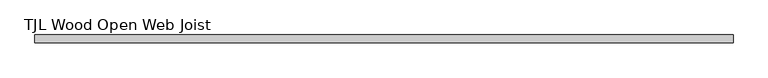
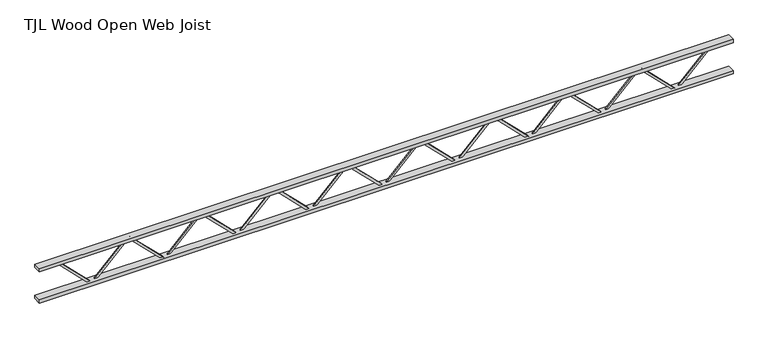
"""IFC4 building model written with IfcOpenShell, lengths in millimetres: beam geometry, TJL Wood Open Web Joist."""

from ifc_helpers import new_model, si_unit, frame, origin, place, context, project, spatial, polyline, outline, extrude, source, transform, mapped, element, save


def tjl_wood_open_web_joist_31244e6a(model_context):
    return source(origin(), model_context, "Body", "SweptSolid", [
        extrude(outline(polyline([(171.45, 2860.2340278), (196.85, 2860.2340278), (196.85, 2842.2957039), (-171.45, 2471.7908428), (-171.45, 2426.2291667), (-196.85, 2426.2291667), (-196.85, 2482.2674905), (171.45, 2852.7723517), (171.45, 2860.2340278)])), frame((0.0, 0.0, 0.0), z_axis=(0.0, 1.0, 0.0), x_axis=(0.0, 0.0, 1.0)), (0.0, 0.0, 1.0), 12.7),
        extrude(outline(polyline([(196.85, 2043.0243056), (171.45, 2043.0243056), (171.45, 2050.4859817), (-196.85, 2420.9908428), (-196.85, 2477.0291667), (-171.45, 2477.0291667), (-171.45, 2431.4674905), (196.85, 2060.9626294), (196.85, 2043.0243056)])), frame((0.0, -12.7, 0.0), z_axis=(0.0, 1.0, 0.0), x_axis=(0.0, 0.0, 1.0)), (0.0, 0.0, 1.0), 12.7),
        extrude(outline(polyline([(171.45, 2043.0243056), (196.85, 2043.0243056), (196.85, 2025.0859817), (-171.45, 1654.5811206), (-171.45, 1609.0194444), (-196.85, 1609.0194444), (-196.85, 1665.0577683), (171.45, 2035.5626294), (171.45, 2043.0243056)])), frame((0.0, 0.0, 0.0), z_axis=(0.0, 1.0, 0.0), x_axis=(0.0, 0.0, 1.0)), (0.0, 0.0, 1.0), 12.7),
        extrude(outline(polyline([(196.85, 1225.8145833), (171.45, 1225.8145833), (171.45, 1233.2762595), (-196.85, 1603.7811206), (-196.85, 1659.8194444), (-171.45, 1659.8194444), (-171.45, 1614.2577683), (196.85, 1243.7529072), (196.85, 1225.8145833)])), frame((0.0, -12.7, 0.0), z_axis=(0.0, 1.0, 0.0), x_axis=(0.0, 0.0, 1.0)), (0.0, 0.0, 1.0), 12.7),
        extrude(outline(polyline([(171.45, 1225.8145833), (196.85, 1225.8145833), (196.85, 1207.8762595), (-171.45, 837.3713983), (-171.45, 791.8097222), (-196.85, 791.8097222), (-196.85, 847.8480461), (171.45, 1218.3529072), (171.45, 1225.8145833)])), frame((0.0, 0.0, 0.0), z_axis=(0.0, 1.0, 0.0), x_axis=(0.0, 0.0, 1.0)), (0.0, 0.0, 1.0), 12.7),
        extrude(outline(polyline([(196.85, 408.6048611), (171.45, 408.6048611), (171.45, 416.0665372), (-196.85, 786.5713983), (-196.85, 842.6097222), (-171.45, 842.6097222), (-171.45, 797.0480461), (196.85, 426.543185), (196.85, 408.6048611)])), frame((0.0, -12.7, 0.0), z_axis=(0.0, 1.0, 0.0), x_axis=(0.0, 0.0, 1.0)), (0.0, 0.0, 1.0), 12.7),
        extrude(outline(polyline([(171.45, 408.6048611), (196.85, 408.6048611), (196.85, 390.6665372), (-171.45, 20.1616761), (-171.45, -25.4), (-196.85, -25.4), (-196.85, 30.6383239), (171.45, 401.143185), (171.45, 408.6048611)])), frame((0.0, 0.0, 0.0), z_axis=(0.0, 1.0, 0.0), x_axis=(0.0, 0.0, 1.0)), (0.0, 0.0, 1.0), 12.7),
        extrude(outline(polyline([(196.85, -408.6048611), (171.45, -408.6048611), (171.45, -401.143185), (-196.85, -30.6383239), (-196.85, 25.4), (-171.45, 25.4), (-171.45, -20.1616761), (196.85, -390.6665372), (196.85, -408.6048611)])), frame((0.0, -12.7, 0.0), z_axis=(0.0, 1.0, 0.0), x_axis=(0.0, 0.0, 1.0)), (0.0, 0.0, 1.0), 12.7),
        extrude(outline(polyline([(171.45, -408.6048611), (196.85, -408.6048611), (196.85, -426.543185), (-171.45, -797.0480461), (-171.45, -842.6097222), (-196.85, -842.6097222), (-196.85, -786.5713983), (171.45, -416.0665372), (171.45, -408.6048611)])), frame((0.0, 0.0, 0.0), z_axis=(0.0, 1.0, 0.0), x_axis=(0.0, 0.0, 1.0)), (0.0, 0.0, 1.0), 12.7),
        extrude(outline(polyline([(196.85, -1225.8145833), (171.45, -1225.8145833), (171.45, -1218.3529072), (-196.85, -847.8480461), (-196.85, -791.8097222), (-171.45, -791.8097222), (-171.45, -837.3713983), (196.85, -1207.8762595), (196.85, -1225.8145833)])), frame((0.0, -12.7, 0.0), z_axis=(0.0, 1.0, 0.0), x_axis=(0.0, 0.0, 1.0)), (0.0, 0.0, 1.0), 12.7),
        extrude(outline(polyline([(171.45, -1225.8145833), (196.85, -1225.8145833), (196.85, -1243.7529072), (-171.45, -1614.2577683), (-171.45, -1659.8194444), (-196.85, -1659.8194444), (-196.85, -1603.7811206), (171.45, -1233.2762595), (171.45, -1225.8145833)])), frame((0.0, 0.0, 0.0), z_axis=(0.0, 1.0, 0.0), x_axis=(0.0, 0.0, 1.0)), (0.0, 0.0, 1.0), 12.7),
        extrude(outline(polyline([(196.85, -2043.0243056), (171.45, -2043.0243056), (171.45, -2035.5626294), (-196.85, -1665.0577683), (-196.85, -1609.0194444), (-171.45, -1609.0194444), (-171.45, -1654.5811206), (196.85, -2025.0859817), (196.85, -2043.0243056)])), frame((0.0, -12.7, 0.0), z_axis=(0.0, 1.0, 0.0), x_axis=(0.0, 0.0, 1.0)), (0.0, 0.0, 1.0), 12.7),
        extrude(outline(polyline([(171.45, -2043.0243056), (196.85, -2043.0243056), (196.85, -2060.9626294), (-171.45, -2431.4674905), (-171.45, -2477.0291667), (-196.85, -2477.0291667), (-196.85, -2420.9908428), (171.45, -2050.4859817), (171.45, -2043.0243056)])), frame((0.0, 0.0, 0.0), z_axis=(0.0, 1.0, 0.0), x_axis=(0.0, 0.0, 1.0)), (0.0, 0.0, 1.0), 12.7),
        extrude(outline(polyline([(196.85, -2860.2340278), (171.45, -2860.2340278), (171.45, -2852.7723517), (-196.85, -2482.2674905), (-196.85, -2426.2291667), (-171.45, -2426.2291667), (-171.45, -2471.7908428), (196.85, -2842.2957039), (196.85, -2860.2340278)])), frame((0.0, -12.7, 0.0), z_axis=(0.0, 1.0, 0.0), x_axis=(0.0, 0.0, 1.0)), (0.0, 0.0, 1.0), 12.7),
        extrude(outline(polyline([(171.45, 3677.44375), (196.85, 3677.44375), (196.85, 3659.5054261), (-171.45, 3289.000565), (-171.45, 3243.4388889), (-196.85, 3243.4388889), (-196.85, 3299.4772128), (171.45, 3669.9820739), (171.45, 3677.44375)])), frame((0.0, 0.0, 0.0), z_axis=(0.0, 1.0, 0.0), x_axis=(0.0, 0.0, 1.0)), (0.0, 0.0, 1.0), 12.7),
        extrude(outline(polyline([(196.85, 2860.2340278), (171.45, 2860.2340278), (171.45, 2867.6957039), (-196.85, 3238.200565), (-196.85, 3294.2388889), (-171.45, 3294.2388889), (-171.45, 3248.6772128), (196.85, 2878.1723517), (196.85, 2860.2340278)])), frame((0.0, -12.7, 0.0), z_axis=(0.0, 1.0, 0.0), x_axis=(0.0, 0.0, 1.0)), (0.0, 0.0, 1.0), 12.7),
        extrude(outline(polyline([(171.45, -2860.2340278), (196.85, -2860.2340278), (196.85, -2878.1723517), (-171.45, -3248.6772128), (-171.45, -3294.2388889), (-196.85, -3294.2388889), (-196.85, -3238.200565), (171.45, -2867.6957039), (171.45, -2860.2340278)])), frame((0.0, 0.0, 0.0), z_axis=(0.0, 1.0, 0.0), x_axis=(0.0, 0.0, 1.0)), (0.0, 0.0, 1.0), 12.7),
        extrude(outline(polyline([(196.85, -3677.44375), (171.45, -3677.44375), (171.45, -3669.9820739), (-196.85, -3299.4772128), (-196.85, -3243.4388889), (-171.45, -3243.4388889), (-171.45, -3289.000565), (196.85, -3659.5054261), (196.85, -3677.44375)])), frame((0.0, -12.7, 0.0), z_axis=(0.0, 1.0, 0.0), x_axis=(0.0, 0.0, 1.0)), (0.0, 0.0, 1.0), 12.7),
        extrude(outline(polyline([(3880.64375, 44.45), (3880.64375, -44.45), (-3880.64375, -44.45), (-3880.64375, 44.45), (3880.64375, 44.45)])), frame((0.0, 0.0, 165.1), z_axis=(0.0, 0.0, 1.0), x_axis=(1.0, 0.0, 0.0)), (0.0, 0.0, 1.0), 38.1),
        extrude(outline(polyline([(3880.64375, 44.45), (3880.64375, -44.45), (-3880.64375, -44.45), (-3880.64375, 44.45), (3880.64375, 44.45)])), frame((0.0, 0.0, -203.2), z_axis=(0.0, 0.0, 1.0), x_axis=(1.0, 0.0, 0.0)), (0.0, 0.0, 1.0), 38.1),
    ])


if __name__ == "__main__":
    model = new_model("IFC4")
    model_context = context("Model", 3, world=origin())
    ifc_project = project(units=[si_unit("LENGTHUNIT", "METRE", prefix="MILLI")], contexts=[model_context])
    site = spatial("IfcSite", under=ifc_project)
    building = spatial("IfcBuilding", under=site)
    placement = place(None, origin())
    tjl_wood_open_web_joist_shape = tjl_wood_open_web_joist_31244e6a(model_context)
    element("IfcBeam", 1, ObjectType="TJL Wood Open Web Joist : 16\" PREENGINEERED FLOOR TRUSS", at=placement, inside=building, context=model_context, shape_type="MappedRepresentation", body=[
        mapped(tjl_wood_open_web_joist_shape, transform((0.0, 0.0, 0.0), x_axis=(1.0, 0.0, 0.0), y_axis=(0.0, 1.0, 0.0), z_axis=(0.0, 0.0, 1.0))),
    ])
    save(model, "model.ifc")

# Revit data of these elements
# Type "TJL Wood Open Web Joist : 16\" PREENGINEERED FLOOR TRUSS"
#   Web Thickness = 0' - 1"
#   Web Leg = 0' - 1"
#   Start Offset [instance default] = 0' - 0"
#   Top Chord Start Extension [instance default] = 0' - 0"
#   PanelArrayLength [instance default] = 22' - 8"
#   Depth = 1' - 4"
#   PanelWidth [instance default] = 2' - 6.22222"
#   Offset Length 2 [instance default] = 0' - 8"
#   Offset Length 1 [instance default] = 0' - 8"
#   End Panel [instance default] = 0' - 8"
#   End Offset [instance default] = 0' - 0"
#   Top Chord End Extension [instance default] = 0' - 0"
#   Chord Width = 0' - 3 1/2"
#   Chord Depth = 0' - 1 1/2"
#   Bottom Chord Start Extension [instance default] = 0' - 0"
#   Bottom Chord End Extension [instance default] = 0' - 0"
#   Length [instance default] = 24' - 0"
#   PanelArrayNum [instance default] = 9
#   Web Rendering Material = none
#   Structural Material = none
#   Assembly Code = ""
# Element 1 (IfcBeam, "TJL Wood Open Web Joist : 16\" PREENGINEERED FLOOR TRUSS")
#   PanelArrayLength = 24' - 1 9/16"
#   PanelWidth = 2' - 8.17361"
